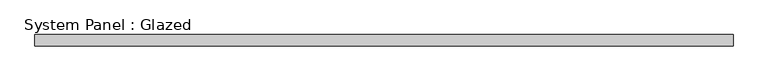
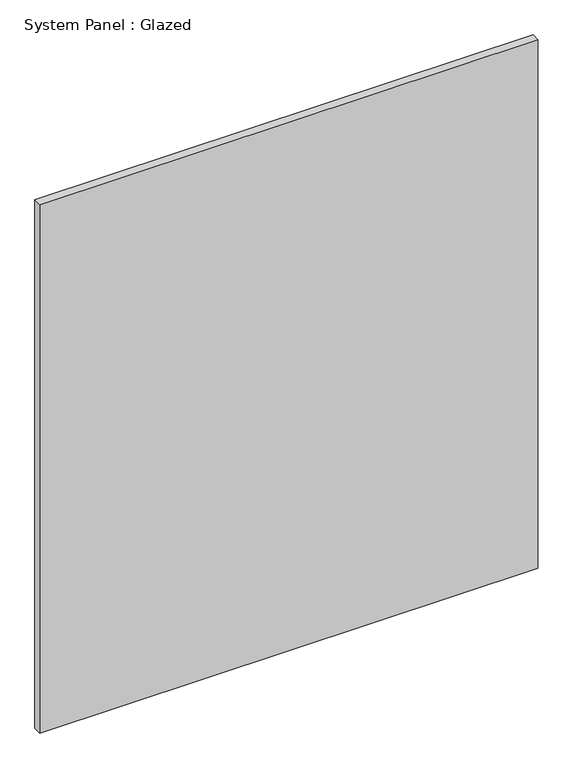
"""IFC4 building model written with IfcOpenShell, lengths in millimetres: plate geometry, System Panel : Glazed."""

from ifc_helpers import new_model, si_unit, origin, origin_with_axes, place, context, project, spatial, polyline, outline, extrude, source, transform, mapped, element, save


def system_panel_glazed_f8206a69(model_context):
    return source(origin(), model_context, "Body", "SweptSolid", [
        extrude(outline(polyline([(757.5465291, 24.5), (-757.5465291, 24.5), (-757.5465291, 49.5), (757.5465291, 49.5), (757.5465291, 24.5)])), origin_with_axes(), (0.0, 0.0, 1.0), 1699.4222628),
    ])


if __name__ == "__main__":
    model = new_model("IFC4")
    model_context = context("Model", 3, world=origin())
    ifc_project = project(units=[si_unit("LENGTHUNIT", "METRE", prefix="MILLI")], contexts=[model_context])
    site = spatial("IfcSite", under=ifc_project)
    building = spatial("IfcBuilding", under=site)
    placement = place(None, origin())
    system_panel_glazed_shape = system_panel_glazed_f8206a69(model_context)
    element("IfcPlate", 1, ObjectType="System Panel : Glazed", at=placement, inside=building, context=model_context, shape_type="MappedRepresentation", body=[
        mapped(system_panel_glazed_shape, transform((0.0, 0.0, 0.0), x_axis=(1.0, 0.0, 0.0), y_axis=(0.0, 1.0, 0.0), z_axis=(0.0, 0.0, 1.0))),
    ])
    save(model, "model.ifc")

# Revit data of these elements
# Element 1 (IfcPlate, "System Panel : Glazed")
#   Materials on its faces: "Glass"
# Materials
#   "Glass": class "Glass", colour RGB 218 227 224, transparency 0.85, Description = "Soda Lime Glass", Cost = 0
